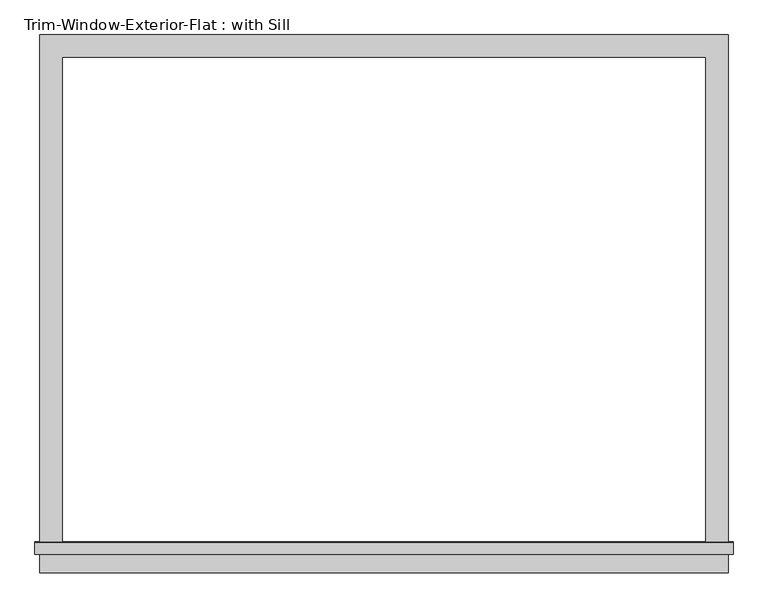
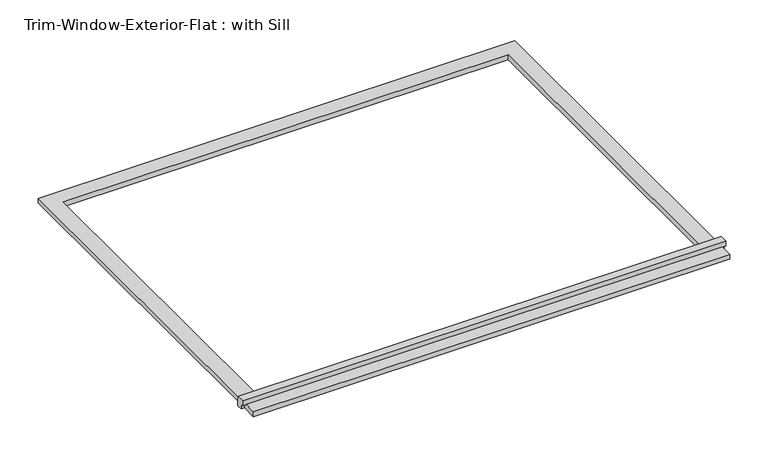
"""IFC4 building model written with IfcOpenShell, lengths in millimetres: proxy geometry, Trim-Window-Exterior-Flat : with Sill."""

from ifc_helpers import new_model, si_unit, frame, origin, origin_with_axes, place, context, project, spatial, polyline, outline, extrude, source, transform, mapped, element, save


def trim_window_exterior_flat_with_sill_12820e37(model_context):
    return source(origin(), model_context, "Body", "SweptSolid", [
        extrude(outline(polyline([(882.65, -1266.7823709), (882.65, -1323.9323709), (-882.65, -1323.9323709), (-882.65, -1266.7823709), (882.65, -1266.7823709)])), origin_with_axes(), (0.0, 0.0, 1.0), 19.05),
        extrude(outline(polyline([(-1276.35, 38.1), (-1247.0580645, 38.1), (-1244.6, 19.05), (-1244.6, 0.0), (-1266.7823709, 0.0), (-1266.7823709, 19.05), (-1276.35, 19.05), (-1276.35, 38.1)])), frame((-895.35, 0.0, 0.0), z_axis=(1.0, 0.0, 0.0), x_axis=(0.0, 1.0, 0.0)), (0.0, 0.0, 1.0), 1790.7),
        extrude(outline(polyline([(-882.65, 57.15), (882.65, 57.15), (882.65, -1244.6), (825.5, -1244.6), (825.5, 0.0), (-825.5, 0.0), (-825.5, -1244.6), (-882.65, -1244.6), (-882.65, 57.15)])), origin_with_axes(), (0.0, 0.0, 1.0), 19.05),
    ])


if __name__ == "__main__":
    model = new_model("IFC4")
    model_context = context("Model", 3, world=origin())
    ifc_project = project(units=[si_unit("LENGTHUNIT", "METRE", prefix="MILLI")], contexts=[model_context])
    site = spatial("IfcSite", under=ifc_project)
    building = spatial("IfcBuilding", under=site)
    placement = place(None, origin())
    trim_window_exterior_flat_with_sill_shape = trim_window_exterior_flat_with_sill_12820e37(model_context)
    element("IfcBuildingElementProxy", 1, Name="Trim-Window-Exterior-Flat : with Sill", ObjectType="Trim-Window-Exterior-Flat : with Sill", at=placement, inside=building, context=model_context, shape_type="MappedRepresentation", body=[
        mapped(trim_window_exterior_flat_with_sill_shape, transform((0.0, 0.0, 0.0), x_axis=(1.0, 0.0, 0.0), y_axis=(0.0, 1.0, 0.0), z_axis=(0.0, 0.0, 1.0))),
    ])
    save(model, "model.ifc")

# Revit data of these elements
# Type "Trim-Window-Exterior-Flat : with Sill"
#   Trim Width = 0' - 2 1/4"
#   Trim Thickness_Picture Frame = 0' - 1 1/4"
#   Trim Thickness_with Sill = 0' - 0 3/4"
#   Sill Thickness = 0' - 1 1/4"
#   Opening Width [instance default] = 2' - 0"
#   Opening Height [instance default] = 3' - 0"
#   Default Elevation = 4' - 0"
#   Sill = yes
#   Picture Frame = no
#   Trim Material [instance default] = none
# Element 1 (IfcBuildingElementProxy, "Trim-Window-Exterior-Flat : with Sill")
#   Opening Width = 5' - 5"
#   Opening Height = 4' - 1"
#   Trim Material = 1X WOOD COMPOSITE TRIM
#   Materials on its faces: "1X WOOD COMPOSITE TRIM"
# Materials
#   "1X WOOD COMPOSITE TRIM": class "Generic", colour RGB 88 61 61, transparency 0, Cost = 0
